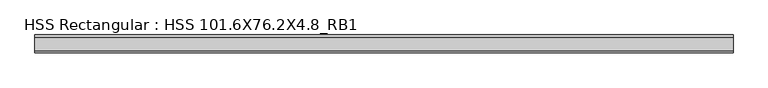
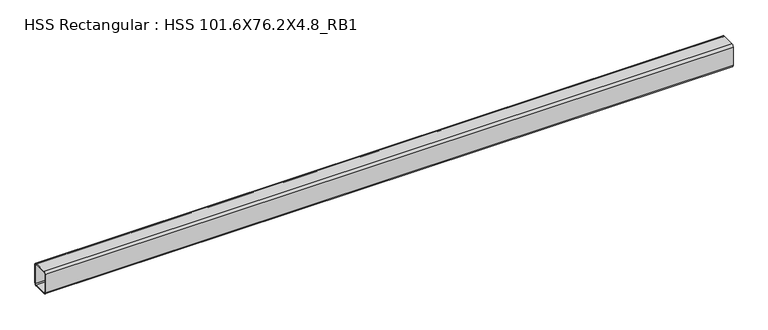
"""IFC4 building model written with IfcOpenShell, lengths in millimetres: beam geometry, HSS Rectangular : HSS 101.6X76.2X4.8_RB1."""

from ifc_helpers import new_model, si_unit, point, frame, frame_2d, origin, place, context, project, spatial, polyline, circle_curve, trimmed, segment, composite_curve, outline, extrude, source, transform, mapped, element, save


def hss_rectangular_hss_101_6x76_2x4_8_rb1_f8706a1e(model_context):
    return source(origin(), model_context, "Body", "SweptSolid", [
        extrude(outline(composite_curve([segment(polyline([(38.1, 41.275), (38.1, -41.275)]), True, "CONTINUOUS"), segment(trimmed(circle_curve(frame_2d((28.575, -41.275)), 9.525), [point((38.1, -41.275))], [point((28.575, -50.8))], False, "CARTESIAN"), True, "CONTINUOUS"), segment(polyline([(28.575, -50.8), (-28.575, -50.8)]), True, "CONTINUOUS"), segment(trimmed(circle_curve(frame_2d((-28.575, -41.275)), 9.525), [point((-28.575, -50.8))], [point((-38.1, -41.275))], False, "CARTESIAN"), True, "CONTINUOUS"), segment(polyline([(-38.1, -41.275), (-38.1, 41.275)]), True, "CONTINUOUS"), segment(trimmed(circle_curve(frame_2d((-28.575, 41.275)), 9.525), [point((-38.1, 41.275))], [point((-28.575, 50.8))], False, "CARTESIAN"), True, "CONTINUOUS"), segment(polyline([(-28.575, 50.8), (28.575, 50.8)]), True, "CONTINUOUS"), segment(trimmed(circle_curve(frame_2d((28.575, 41.275)), 9.525), [point((28.575, 50.8))], [point((38.1, 41.275))], False, "CARTESIAN"), True, "CONTINUOUS")], self_intersect=False), holes=[composite_curve([segment(trimmed(circle_curve(frame_2d((-28.575, 41.275)), 4.7625), [point((-28.575, 46.0375))], [point((-33.3375, 41.275))], True, "CARTESIAN"), True, "CONTINUOUS"), segment(polyline([(-33.3375, 41.275), (-33.3375, -41.275)]), True, "CONTINUOUS"), segment(trimmed(circle_curve(frame_2d((-28.575, -41.275)), 4.7625), [point((-33.3375, -41.275))], [point((-28.575, -46.0375))], True, "CARTESIAN"), True, "CONTINUOUS"), segment(polyline([(-28.575, -46.0375), (28.575, -46.0375)]), True, "CONTINUOUS"), segment(trimmed(circle_curve(frame_2d((28.575, -41.275)), 4.7625), [point((28.575, -46.0375))], [point((33.3375, -41.275))], True, "CARTESIAN"), True, "CONTINUOUS"), segment(polyline([(33.3375, -41.275), (33.3375, 41.275)]), True, "CONTINUOUS"), segment(trimmed(circle_curve(frame_2d((28.575, 41.275)), 4.7625), [point((33.3375, 41.275))], [point((28.575, 46.0375))], True, "CARTESIAN"), True, "CONTINUOUS"), segment(polyline([(28.575, 46.0375), (-28.575, 46.0375)]), True, "CONTINUOUS")], self_intersect=False)]), frame((-1397.2875, 0.0, 0.0), z_axis=(1.0, 0.0, 0.0), x_axis=(0.0, 1.0, 0.0)), (0.0, 0.0, 1.0), 2957.775),
    ])


if __name__ == "__main__":
    model = new_model("IFC4")
    model_context = context("Model", 3, world=origin())
    ifc_project = project(units=[si_unit("LENGTHUNIT", "METRE", prefix="MILLI")], contexts=[model_context])
    site = spatial("IfcSite", under=ifc_project)
    building = spatial("IfcBuilding", under=site)
    placement = place(None, origin())
    hss_rectangular_hss_101_6x76_2x4_8_rb1_shape = hss_rectangular_hss_101_6x76_2x4_8_rb1_f8706a1e(model_context)
    element("IfcBeam", 1, ObjectType="HSS Rectangular : HSS 101.6X76.2X4.8_RB1", at=placement, inside=building, context=model_context, shape_type="MappedRepresentation", body=[
        mapped(hss_rectangular_hss_101_6x76_2x4_8_rb1_shape, transform((0.0, 0.0, 0.0), x_axis=(1.0, 0.0, 0.0), y_axis=(0.0, 1.0, 0.0), z_axis=(0.0, 0.0, 1.0))),
    ])
    save(model, "model.ifc")

# Revit data of these elements
# Type "HSS Rectangular : HSS 101.6X76.2X4.8_RB1"
#   Section Name Key = "HSS 4X3X3/16"
#   Assembly Code = "B10"
#   Width = 7.62 cm
#   Wall Nominal Thickness = 0.4763 cm
#   Wall Design Thickness = 0.442 cm
#   Torsional Moment of Inertia = 260.561 cm⁴
#   Torsional Modulus = 61.2876 cm³
#   Section Area = 14.4516 cm²
#   Plastic Modulus weak axis = 40.3122 cm³
#   Plastic Modulus strong axis = 49.1612 cm³
#   Perimeter = 0.881482 m²/m
#   Outer Fillet = 0.9525 cm
#   Nominal Weight = 12.1285 kgf/m
#   Moment of Inertia weak axis = 131.529 cm⁴
#   Moment of Inertia strong axis = 205.202 cm⁴
#   Inner Fillet = 0.4763 cm
#   Height = 10.16 cm
#   Elastic Modulus weak axis = 34.4128 cm³
#   Elastic Modulus strong axis = 40.476 cm³
#   Centroid Vertical = 5.08 cm
#   Centroid Horizontal = 3.81 cm
#   Length [instance default] = 1524 mm
#   Structural Material [instance default] = Steel ASTM A500, Grade B, Rectangular and Square
#   Principal Axes Angle = 0
# Element 1 (IfcBeam, "HSS Rectangular : HSS 101.6X76.2X4.8_RB1")
#   Structural Material = Steel ASTM A992
#   Materials on its faces: "Steel ASTM A992"
# Materials
#   "Steel ASTM A500, Grade B, Rectangular and Square": class "Metal", colour RGB 199 199 199, transparency 0, Description = "Carbon steel", Cost = 0
#   "Steel ASTM A992": class "Metal", colour RGB 199 199 199, transparency 0, Description = "Structural steel 50ksi", Cost = 0
